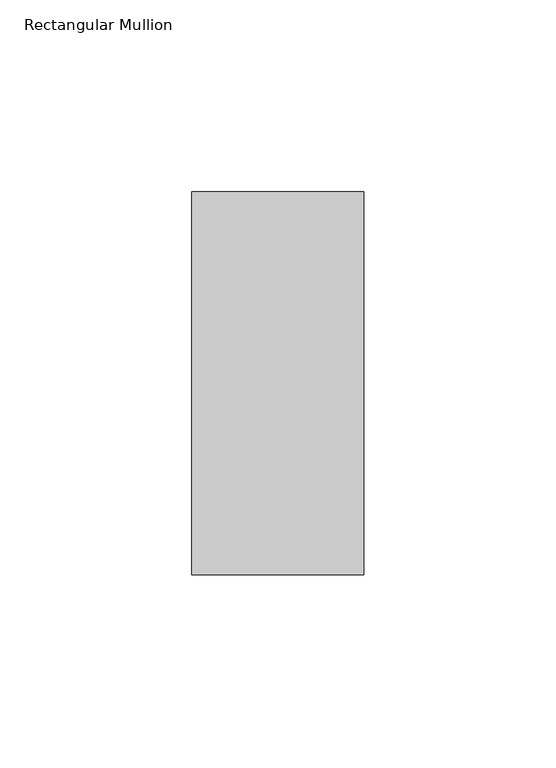
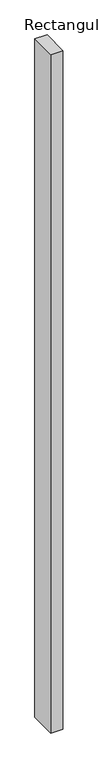
"""IFC4 building model written with IfcOpenShell, lengths in millimetres: member geometry, Rectangular Mullion : 알루미늄_Rectangular Cap_100 x 45."""

from ifc_helpers import new_model, si_unit, frame, origin, place, context, project, spatial, polyline, outline, extrude, source, transform, mapped, element, save


def rectangular_mullion_121cf21c(model_context):
    return source(origin(), model_context, "Body", "SweptSolid", [
        extrude(outline(polyline([(0.0, 50.0), (0.0, -50.0), (-45.0, -50.0), (-45.0, 50.0), (0.0, 50.0)])), frame((0.0, 0.0, -2625.0), z_axis=(0.0, 0.0, 1.0), x_axis=(1.0, 0.0, 0.0)), (0.0, 0.0, 1.0), 2625.0),
    ])


if __name__ == "__main__":
    model = new_model("IFC4")
    model_context = context("Model", 3, world=origin())
    ifc_project = project(units=[si_unit("LENGTHUNIT", "METRE", prefix="MILLI")], contexts=[model_context])
    site = spatial("IfcSite", under=ifc_project)
    building = spatial("IfcBuilding", under=site)
    placement = place(None, origin())
    rectangular_mullion_shape = rectangular_mullion_121cf21c(model_context)
    element("IfcMember", 1, ObjectType="Rectangular Mullion : 알루미늄_Rectangular Cap_100 x 45", at=placement, inside=building, context=model_context, shape_type="MappedRepresentation", body=[
        mapped(rectangular_mullion_shape, transform((0.0, 0.0, 0.0), x_axis=(1.0, 0.0, 0.0), y_axis=(0.0, 1.0, 0.0), z_axis=(0.0, 0.0, 1.0))),
    ])
    save(model, "model.ifc")

# Revit data of these elements
# Type "Rectangular Mullion : 알루미늄_Rectangular Cap_100 x 45"
#   built-in parameter 1007304 = 0.328084 (stored number, unit not read)
#   built-in parameter 1007301 = 0.0738189 (stored number, unit not read)
#   built-in parameter 1007300 = 0.0738189 (stored number, unit not read)
# Element 1 (IfcMember, "Rectangular Mullion : 알루미늄_Rectangular Cap_100 x 45")
#   Materials on its faces: "00_Metal_Stainless Steel"
# Materials
#   "00_Metal_Stainless Steel": class "Metal", colour RGB 148 148 148, transparency 0, Description = "Steel", Cost = 0
